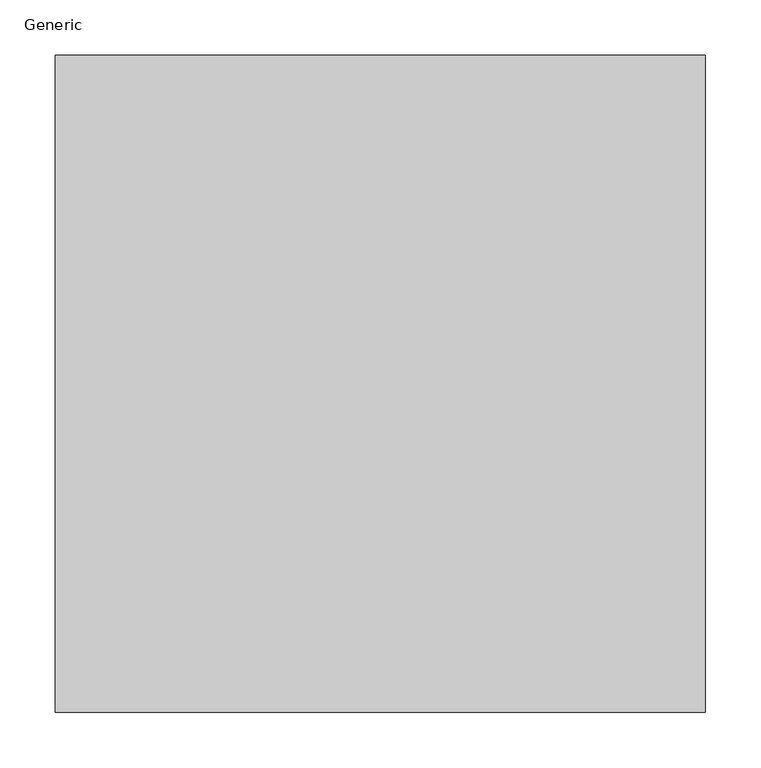
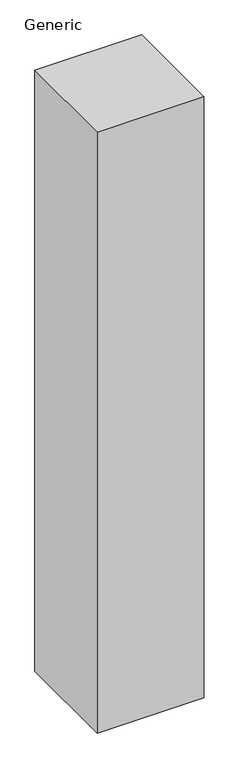
"""IFC4 building model written with IfcOpenShell, lengths in millimetres: column geometry, WWm-ConcreteRectangular-Instance : Generic."""

from ifc_helpers import new_model, si_unit, frame, origin, place, context, project, spatial, polyline, outline, extrude, source, transform, mapped, element, save


def generic_c36b0d2a(model_context):
    return source(origin(), model_context, "Body", "SweptSolid", [
        extrude(outline(polyline([(283.4553773, 289.5868214), (283.4553773, -304.8), (-304.8, -304.8), (-304.8, 289.5868214), (283.4553773, 289.5868214)])), frame((0.0, 0.0, 10500.0), z_axis=(0.0, 0.0, 1.0), x_axis=(1.0, 0.0, 0.0)), (0.0, 0.0, 1.0), 3500.0),
    ])


if __name__ == "__main__":
    model = new_model("IFC4")
    model_context = context("Model", 3, world=origin())
    ifc_project = project(units=[si_unit("LENGTHUNIT", "METRE", prefix="MILLI")], contexts=[model_context])
    site = spatial("IfcSite", under=ifc_project)
    building = spatial("IfcBuilding", under=site)
    placement = place(None, origin())
    generic_shape = generic_c36b0d2a(model_context)
    element("IfcColumn", 1, ObjectType="WWm-ConcreteRectangular-Instance : Generic", at=placement, inside=building, context=model_context, shape_type="MappedRepresentation", body=[
        mapped(generic_shape, transform((0.0, 0.0, 0.0), x_axis=(1.0, 0.0, 0.0), y_axis=(0.0, 1.0, 0.0), z_axis=(0.0, 0.0, 1.0))),
    ])
    save(model, "model.ifc")

# Revit data of these elements
# Type "WWm-ConcreteRectangular-Instance : Generic"
#   Depth [instance default] = 600 mm
#   Offset Base = 0 mm
#   Offset Top = 0 mm
#   Width [instance default] = 600 mm
#   Material = WW-EC-CR-CastInPlace
#   Assembly Code = ""
# Element 1 (IfcColumn, "WWm-ConcreteRectangular-Instance : Generic")
#   Depth = 594.387 mm
#   Width = 588.255 mm
#   Materials on its faces: "WW-EC-CR-CastInPlace"
# Materials
#   "WW-EC-CR-CastInPlace": class "Concrete", colour RGB 255 255 255, transparency 0, Comments = "If region requests all-white model, remove image from asset", Description = "Cast in Place Concrete", Cost = 0
